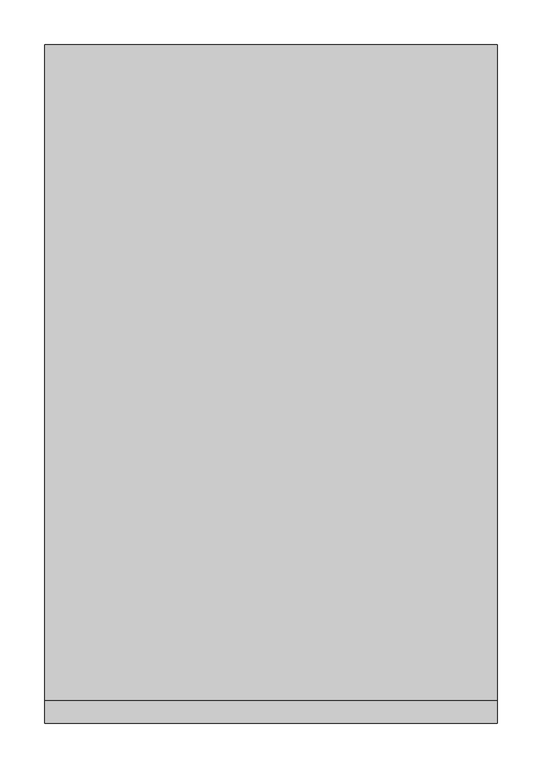
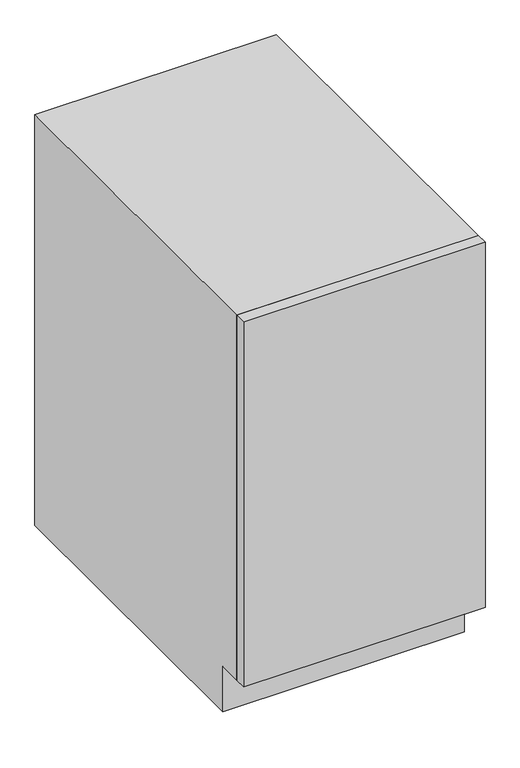
"""IFC4 building model written with IfcOpenShell, lengths in millimetres: furniture geometry, OD_CW_Base Cabinet : OD_CW_Base Cabinet."""

from ifc_helpers import new_model, si_unit, frame, origin, place, context, project, spatial, polyline, outline, extrude, source, transform, mapped, element, save


def furniture_9e1ca412(model_context):
    return source(origin(), model_context, "Body", "SweptSolid", [
        extrude(outline(polyline([(18.7377049, -127.0), (526.7377049, -127.0), (526.7377049, -152.4), (18.7377049, -152.4), (18.7377049, -127.0)])), frame((0.0, 0.0, 101.6), z_axis=(0.0, 0.0, 1.0), x_axis=(1.0, 0.0, 0.0)), (0.0, 0.0, 1.0), 812.8),
        extrude(outline(polyline([(-127.0, 914.4), (609.6, 914.4), (609.6, 0.0), (-76.2, 0.0), (-76.2, 101.6), (-127.0, 101.6), (-127.0, 914.4)])), frame((18.7377049, 0.0, 0.0), z_axis=(1.0, 0.0, 0.0), x_axis=(0.0, 1.0, 0.0)), (0.0, 0.0, 1.0), 508.0),
    ])


if __name__ == "__main__":
    model = new_model("IFC4")
    model_context = context("Model", 3, world=origin())
    ifc_project = project(units=[si_unit("LENGTHUNIT", "METRE", prefix="MILLI")], contexts=[model_context])
    site = spatial("IfcSite", under=ifc_project)
    building = spatial("IfcBuilding", under=site)
    placement = place(None, origin())
    furniture_shape = furniture_9e1ca412(model_context)
    element("IfcFurniture", 1, ObjectType="OD_CW_Base Cabinet : OD_CW_Base Cabinet", at=placement, inside=building, context=model_context, shape_type="MappedRepresentation", body=[
        mapped(furniture_shape, transform((0.0, 0.0, 0.0), x_axis=(1.0, 0.0, 0.0), y_axis=(0.0, 1.0, 0.0), z_axis=(0.0, 0.0, 1.0))),
    ])
    save(model, "model.ifc")

# Revit data of these elements
# Type "OD_CW_Base Cabinet : OD_CW_Base Cabinet"
#   OD_CW_Width [instance default] = 2' - 10"
#   OD_CW_Length [instance default] = 8' - 0"
#   OD_CW_Height [instance default] = 2' - 3"
#   Depth = 2' - 0"
#   Height = 3' - 0"
#   Width = 4' - 0"
#   OD_CW_Material_Front Panel [instance default] = none
#   OD_CW_Material_Body [instance default] = none
# Element 1 (IfcFurniture, "OD_CW_Base Cabinet : OD_CW_Base Cabinet")
#   OD_CW_Width = 2' - 6"
#   OD_CW_Length = 1' - 8"
#   OD_CW_Height = 3' - 0"
#   OD_CW_Material_Body = DIVIDER ROUNDER
#   Materials on its faces: "DIVIDER ROUNDER", "CASEWORK"
# Materials
#   "DIVIDER ROUNDER": class "Generic", colour RGB 187 187 187, transparency 0, Cost = 0
#   "CASEWORK": class "Generic", colour RGB 181 181 181, transparency 0, Cost = 0
